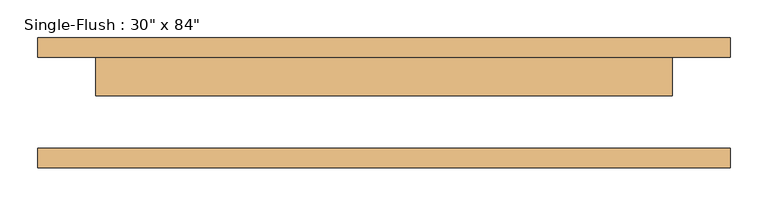
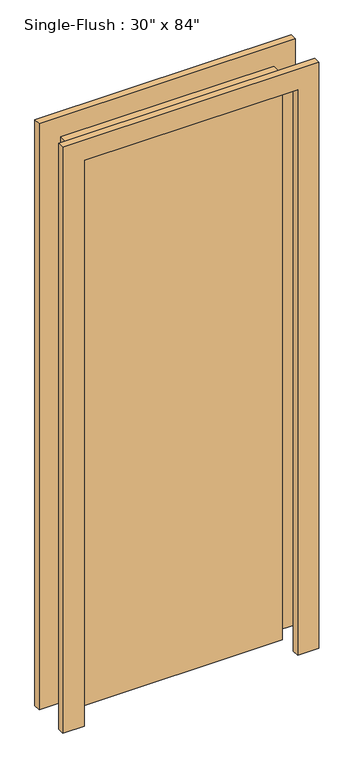
"""IFC4 building model written with IfcOpenShell, lengths in millimetres: door geometry."""

import ifcopenshell
import ifcopenshell.guid

model = None  # the IFC model being written
_history = None  # IfcOwnerHistory: only IFC2X3 demands one
_inside = {}  # id of a spatial element -> (the spatial element, [elements in it])
_under = {}  # id of a project, library or spatial element -> (it, [spatial elements below it])
_declared = {}  # id of a project -> (the project, [libraries it declares])
_typed = {}  # id of a type object -> (the type object, [elements of that type])
_made_of = {}  # id of a material, layer set ... -> (it, [elements and type objects made of it])


def new_model(schema):
    """Start an empty IFC model of exactly this schema.

    Asked for "IFC4X3", IfcOpenShell would pick the latest addendum, in which some entities
    have other attributes; the version numbers below select the first issue.
    IFC2X3 requires an IfcOwnerHistory on every rooted entity: one is made here for all.
    """
    global model, _history
    if schema == "IFC4X3":
        model = ifcopenshell.file(schema_version=(4, 3, 0, 0))
    else:
        model = ifcopenshell.file(schema=schema)
    _inside.clear()
    _under.clear()
    _declared.clear()
    _typed.clear()
    _made_of.clear()
    _history = None
    if model.schema == "IFC2X3":
        org = make("IfcOrganization", Name="unknown")
        user = make(
            "IfcPersonAndOrganization",
            ThePerson=make("IfcPerson", FamilyName="unknown"),
            TheOrganization=org,
        )
        app = make(
            "IfcApplication",
            ApplicationDeveloper=org,
            Version="unknown",
            ApplicationFullName="unknown",
            ApplicationIdentifier="unknown",
        )
        _history = make(
            "IfcOwnerHistory",
            OwningUser=user,
            OwningApplication=app,
            ChangeAction="ADDED",
            CreationDate=0,
        )
    return model


def make(cls, **values):
    """One entity of the class cls with the attributes given. An attribute that is None is left unset."""
    return model.create_entity(
        cls, **{name: value for name, value in values.items() if value is not None}
    )


def rooted(cls, **values):
    """An entity with a GlobalId (a new one), such as an element, a storey or a relation."""
    return make(cls, GlobalId=ifcopenshell.guid.new(), OwnerHistory=_history, **values)


def si_unit(unit_type, name, prefix=None):
    """IfcSIUnit, for example si_unit("LENGTHUNIT", "METRE", prefix="MILLI")."""
    return make("IfcSIUnit", UnitType=unit_type, Prefix=prefix, Name=name)


def assignment(units):
    """IfcUnitAssignment: the units of a project."""
    return None if units is None else make("IfcUnitAssignment", Units=units)


def point(xyz):
    """IfcCartesianPoint."""
    return None if xyz is None else make("IfcCartesianPoint", Coordinates=xyz)


def direction(xyz):
    """IfcDirection."""
    return None if xyz is None else make("IfcDirection", DirectionRatios=xyz)


def frame(location, z_axis=None, x_axis=None):
    """IfcAxis2Placement3D, a coordinate frame: its origin and axes. An axis left out is left unset."""
    return make(
        "IfcAxis2Placement3D",
        Location=point(location),
        Axis=direction(z_axis),
        RefDirection=direction(x_axis),
    )


def origin():
    """The frame at (0, 0, 0) with its axes left unset."""
    return frame((0.0, 0.0, 0.0))


def origin_with_axes():
    """The frame at (0, 0, 0) with the z axis (0, 0, 1) and the x axis (1, 0, 0) written out."""
    return frame((0.0, 0.0, 0.0), z_axis=(0.0, 0.0, 1.0), x_axis=(1.0, 0.0, 0.0))


def place(relative_to, where):
    """IfcLocalPlacement: puts the frame where relative to a parent placement (None: the world)."""
    return make(
        "IfcLocalPlacement", PlacementRelTo=relative_to, RelativePlacement=where
    )


def context(
    kind, dimensions, precision=None, world=None, true_north=None, identifier=None
):
    """IfcGeometricRepresentationContext, for example the 3D "Model" context."""
    return make(
        "IfcGeometricRepresentationContext",
        ContextIdentifier=identifier,
        ContextType=kind,
        CoordinateSpaceDimension=dimensions,
        Precision=precision,
        WorldCoordinateSystem=world,
        TrueNorth=true_north,
    )


def project(units=None, contexts=None):
    """IfcProject with its units and contexts."""
    return rooted(
        "IfcProject",
        Name="project",
        RepresentationContexts=contexts,
        UnitsInContext=assignment(units),
    )


def spatial(cls, under=None, at=None, **own):
    """A site, building, storey or space (cls), placed at a placement, below another one or the project."""
    s = rooted(cls, ObjectPlacement=at, **own)
    if under is not None:
        _under.setdefault(under.id(), (under, []))[1].append(s)
    return s


def polyline(points):
    """IfcPolyline through the points."""
    return make("IfcPolyline", Points=[point(p) for p in points])


def outline(outer, holes=None, kind="AREA"):
    """IfcArbitraryClosedProfileDef: a profile drawn as a closed curve; with holes, ...WithVoids."""
    if holes is None:
        return make("IfcArbitraryClosedProfileDef", ProfileType=kind, OuterCurve=outer)
    return make(
        "IfcArbitraryProfileDefWithVoids",
        ProfileType=kind,
        OuterCurve=outer,
        InnerCurves=holes,
    )


def extrude(swept, where, along, depth):
    """IfcExtrudedAreaSolid: the profile swept, set in the frame where, extruded along a direction by depth."""
    return make(
        "IfcExtrudedAreaSolid",
        SweptArea=swept,
        Position=where,
        ExtrudedDirection=direction(along),
        Depth=depth,
    )


def shape(context_of_items, identifier, shape_type, items):
    """IfcShapeRepresentation: the items that make up one representation, for example the "Body"."""
    return make(
        "IfcShapeRepresentation",
        ContextOfItems=context_of_items,
        RepresentationIdentifier=identifier,
        RepresentationType=shape_type,
        Items=items,
    )


def source(mapping_origin, context_of_items, identifier, shape_type, items):
    """IfcRepresentationMap: a shape defined once, which mapped items show again and again."""
    return make(
        "IfcRepresentationMap",
        MappingOrigin=mapping_origin,
        MappedRepresentation=shape(context_of_items, identifier, shape_type, items),
    )


def transform(
    local_origin,
    x_axis=None,
    y_axis=None,
    z_axis=None,
    scale=None,
    scale2=None,
    scale3=None,
    uniform=True,
):
    """IfcCartesianTransformationOperator3D, or its non-uniform kind. x_axis, y_axis, z_axis: its Axis1, 2, 3."""
    if uniform:
        return make(
            "IfcCartesianTransformationOperator3D",
            Axis1=direction(x_axis),
            Axis2=direction(y_axis),
            LocalOrigin=point(local_origin),
            Scale=scale,
            Axis3=direction(z_axis),
        )
    return make(
        "IfcCartesianTransformationOperator3DnonUniform",
        Axis1=direction(x_axis),
        Axis2=direction(y_axis),
        LocalOrigin=point(local_origin),
        Scale=scale,
        Axis3=direction(z_axis),
        Scale2=scale2,
        Scale3=scale3,
    )


def mapped(mapping_source, mapping_target):
    """IfcMappedItem: shows the shape of a source again, moved by a transform."""
    return make(
        "IfcMappedItem", MappingSource=mapping_source, MappingTarget=mapping_target
    )


def made_of(thing, what):
    """Note that an element or type object is made of a material, layer set ...; save() writes the relation."""
    if what is not None:
        _made_of.setdefault(what.id(), (what, []))[1].append(thing)
    return thing


def element(
    cls,
    number,
    at=None,
    inside=None,
    cuts=None,
    type_object=None,
    material=None,
    context=None,
    identifier="Body",
    shape_type=None,
    held_by="IfcProductDefinitionShape",
    body=None,
    shapes=None,
    **own,
):
    """One element of the class cls, such as IfcWall. Its Tag is "e" and its number.

    at: its placement. inside: the storey or other place that contains it. cuts: it is an
    opening in that element (IfcRelVoidsElement). A single representation is given by context,
    identifier, shape_type and body (its items); several are given by shapes. held_by: the class
    of the entity that holds the representations. save() writes the other relations.
    """
    e = rooted(cls, Tag="e%d" % number, ObjectPlacement=at, **own)
    if body is not None:
        shapes = [shape(context, identifier, shape_type, body)]
    if shapes is not None:
        e.Representation = make(held_by, Representations=shapes)
    if inside is not None:
        _inside.setdefault(inside.id(), (inside, []))[1].append(e)
    if cuts is not None:
        rooted(
            "IfcRelVoidsElement", RelatingBuildingElement=cuts, RelatedOpeningElement=e
        )
    if type_object is not None:
        _typed.setdefault(type_object.id(), (type_object, []))[1].append(e)
    return made_of(e, material)


def aggregate(whole, parts):
    """IfcRelAggregates: a whole, such as a stair, and the parts it consists of."""
    return rooted("IfcRelAggregates", RelatingObject=whole, RelatedObjects=parts)


def save(model, path):
    """Write the relations noted so far, then the file.

    IfcRelAggregates (storeys below a building ...), IfcRelContainedInSpatialStructure (elements
    in a storey), IfcRelDefinesByType, IfcRelAssociatesMaterial and IfcRelDeclares: one each for
    every whole, place, type object, material and project.
    """
    for whole, parts in _under.values():
        aggregate(whole, parts)
    for where, things in _inside.values():
        rooted(
            "IfcRelContainedInSpatialStructure",
            RelatedElements=things,
            RelatingStructure=where,
        )
    for kind, things in _typed.values():
        rooted("IfcRelDefinesByType", RelatedObjects=things, RelatingType=kind)
    for what, things in _made_of.values():
        rooted("IfcRelAssociatesMaterial", RelatedObjects=things, RelatingMaterial=what)
    for by, libraries in _declared.values():
        rooted("IfcRelDeclares", RelatingContext=by, RelatedDefinitions=libraries)
    model.write(path)


def door_d179b03e(model_context):
    return source(origin(), model_context, "Body", "SweptSolid", [
        extrude(outline(polyline([(2209.8, -457.2), (0.0, -457.2), (0.0, -381.0), (2133.6, -381.0), (2133.6, 381.0), (0.0, 381.0), (0.0, 457.2), (2209.8, 457.2), (2209.8, -457.2)])), frame((0.0, 60.325, 0.0), z_axis=(0.0, 1.0, 0.0), x_axis=(0.0, 0.0, 1.0)), (0.0, 0.0, 1.0), 25.4),
        extrude(outline(polyline([(2209.8, 457.2), (2209.8, -457.2), (0.0, -457.2), (0.0, -381.0), (2133.6, -381.0), (2133.6, 381.0), (0.0, 381.0), (0.0, 457.2), (2209.8, 457.2)])), frame((0.0, -85.725, 0.0), z_axis=(0.0, 1.0, 0.0), x_axis=(0.0, 0.0, 1.0)), (0.0, 0.0, 1.0), 25.4),
        extrude(outline(polyline([(381.0, 9.525), (-381.0, 9.525), (-381.0, 60.325), (381.0, 60.325), (381.0, 9.525)])), origin_with_axes(), (0.0, 0.0, 1.0), 2133.6),
    ])


if __name__ == "__main__":
    model = new_model("IFC4")
    model_context = context("Model", 3, world=origin())
    ifc_project = project(units=[si_unit("LENGTHUNIT", "METRE", prefix="MILLI")], contexts=[model_context])
    site = spatial("IfcSite", under=ifc_project)
    building = spatial("IfcBuilding", under=site)
    placement = place(None, origin())
    door_shape = door_d179b03e(model_context)
    element("IfcDoor", 1, ObjectType="Single-Flush : 30\" x 84\"", at=placement, inside=building, context=model_context, shape_type="MappedRepresentation", body=[
        mapped(door_shape, transform((0.0, 0.0, 0.0), x_axis=(1.0, 0.0, 0.0), y_axis=(0.0, 1.0, 0.0), z_axis=(0.0, 0.0, 1.0))),
    ])
    save(model, "model.ifc")

# Revit data of these elements
# Type "Single-Flush : 30\" x 84\""
#   Type Mark = "4"
#   Construction Type Id = "MDOOR"
#   Assembly Code = "C1020"
#   Analytic Construction = "Metal"
#   Thickness = 0' - 2"
#   Heat Transfer Coefficient (U) = 0.651978 BTU/(h·ft²·°F)
#   Height = 7' - 0"
#   Trim Projection Ext = 0' - 1"
#   Trim Projection Int = 0' - 1"
#   Trim Width = 0' - 3"
#   Width = 2' - 6"
#   Define Thermal Properties by = 1
#   Define Thermal Properties by = 1
#   Door Material = Door - Panel
#   Frame Material = Door - Frame
#   Visual Light Transmittance = 0
#   Solar Heat Gain Coefficient = 0
#   Function = (empty or 0)
#   Wall Closure = (empty or 0)
# Element 1 (IfcDoor, "Single-Flush : 30\" x 84\"")
#   Materials on its faces: "Door - Frame", "Door - Panel"
# Materials
#   "Door - Panel": class "Wood", colour RGB 210 159 95, transparency 0, Cost = 0
#   "Door - Frame": class "Miscellaneous", colour RGB 118 70 51, transparency 0, Cost = 0
